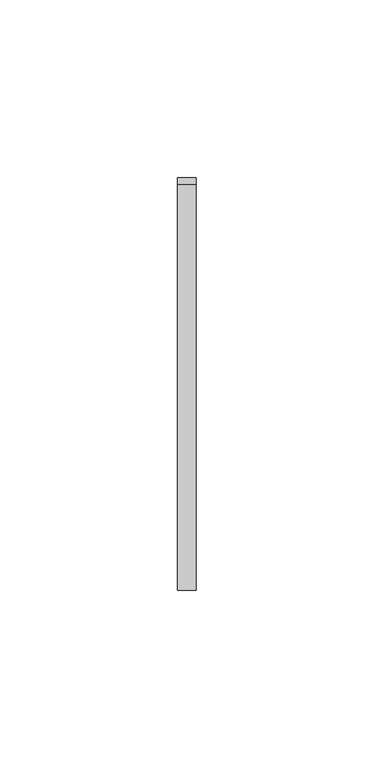
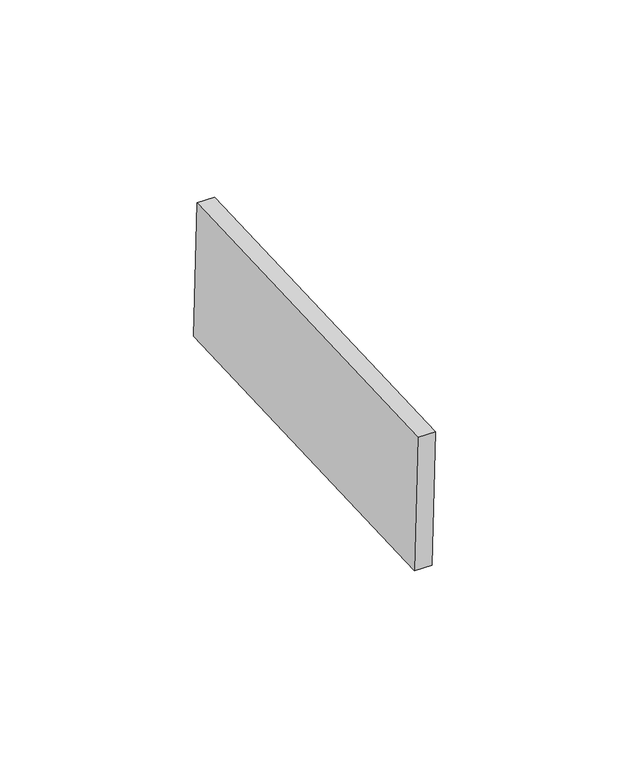
"""IFC4 building model written with IfcOpenShell, lengths in millimetres: proxy geometry, Inner panel:Inner panel:1:Inner panel:1 : Inner panel:Inner panel:300324:2:Inner panel:1:Inner panel:1 : Inner panel:Inner panel:300324:2 : Inner panel:Inner panel:1:Inner panel:1 : Inner panel:Inner panel:300324:300043:77 : Inner panel:Inner panel:1:Inner panel:1 : Inner panel:Inner panel:300324:2:Inner panel:1:Inner panel:1 : Inner panel:Inner panel:300324:2 : Inner panel:Inner panel:1:Inner panel:1 : Inner panel:Inner panel:300324:300043:308120."""

from ifc_helpers import new_model, si_unit, frame, origin, place, context, project, spatial, polyline, outline, extrude, source, transform, mapped, element, save


def generic_models_f36a7794(model_context):
    return source(origin(), model_context, "Body", "SweptSolid", [
        extrude(outline(polyline([(0.0, -114.3), (0.0, 0.0), (5.2138089, 0.0), (5.2138089, -114.3), (0.0, -114.3)])), frame((592717.395117, -578297.797364, 3981.6641254), z_axis=(0.0, -0.04163054471216399, 0.9991330730923527), x_axis=(-1.0, 0.0, 0.0)), (0.0, 0.0, 1.0), 43.2233908),
    ])


if __name__ == "__main__":
    model = new_model("IFC4")
    model_context = context("Model", 3, world=origin())
    ifc_project = project(units=[si_unit("LENGTHUNIT", "METRE", prefix="MILLI")], contexts=[model_context])
    site = spatial("IfcSite", under=ifc_project)
    building = spatial("IfcBuilding", under=site)
    placement = place(None, origin())
    generic_models_shape = generic_models_f36a7794(model_context)
    element("IfcBuildingElementProxy", 1, Name="Inner panel:Inner panel:1:Inner panel:1 : Inner panel:Inner panel:300324:2:Inner panel:1:Inner panel:1 : Inner panel:Inner panel:300324:2 : Inner panel:Inner panel:1:Inner panel:1 : Inner panel:Inner panel:300324:300043:77 : Inner panel:Inner panel:1:Inner panel:1 : Inner panel:Inner panel:300324:2:Inner panel:1:Inner panel:1 : Inner panel:Inner panel:300324:2 : Inner panel:Inner panel:1:Inner panel:1 : Inner panel:Inner panel:300324:300043:308120", ObjectType="Inner panel:Inner panel:1:Inner panel:1 : Inner panel:Inner panel:300324:2:Inner panel:1:Inner panel:1 : Inner panel:Inner panel:300324:2 : Inner panel:Inner panel:1:Inner panel:1 : Inner panel:Inner panel:300324:300043:77 : Inner panel:Inner panel:1:Inner panel:1 : Inner panel:Inner panel:300324:2:Inner panel:1:Inner panel:1 : Inner panel:Inner panel:300324:2 : Inner panel:Inner panel:1:Inner panel:1 : Inner panel:Inner panel:300324:300043:308120", at=placement, inside=building, context=model_context, shape_type="MappedRepresentation", body=[
        mapped(generic_models_shape, transform((0.0, 0.0, 0.0), x_axis=(1.0, 0.0, 0.0), y_axis=(0.0, 1.0, 0.0), z_axis=(0.0, 0.0, 1.0))),
    ])
    save(model, "model.ifc")

# Revit data of these elements
# Type "Inner panel:Inner panel:1:Inner panel:1 : Inner panel:Inner panel:300324:2:Inner panel:1:Inner panel:1 : Inner panel:Inner panel:300324:2 : Inner panel:Inner panel:1:Inner panel:1 : Inner panel:Inner panel:300324:300043:77 : Inner panel:Inner panel:1:Inner panel:1 : Inner panel:Inner panel:300324:2:Inner panel:1:Inner panel:1 : Inner panel:Inner panel:300324:2 : Inner panel:Inner panel:1:Inner panel:1 : Inner panel:Inner panel:300324:300043:308120"
#   NameOverride = "Inner panel:Inner panel:1:Inner panel:1 : Inner panel:Inner panel:300324:2:Inner panel:1:Inner panel:1 : Inner panel:Inner panel:300324:2 : Inner panel:Inner panel:1:Inner panel:1 : Inner panel:Inner panel:300324:300043:308120"
#   ObjectTypeOverride = "Inner panel:1:Inner panel:1 : Inner panel:Inner panel:300324:2 : Inner panel:Inner panel:1:Inner panel:1 : Inner panel:Inner panel:300324:300043"
#   Reference = "Inner panel"
#   Tag = "308120"
# Element 1 (IfcBuildingElementProxy, "Inner panel:Inner panel:1:Inner panel:1 : Inner panel:Inner panel:300324:2:Inner panel:1:Inner panel:1 : Inner panel:Inner panel:300324:2 : Inner panel:Inner panel:1:Inner panel:1 : Inner panel:Inner panel:300324:300043:77 : Inner panel:Inner panel:1:Inner panel:1 : Inner panel:Inner panel:300324:2:Inner panel:1:Inner panel:1 : Inner panel:Inner panel:300324:2 : Inner panel:Inner panel:1:Inner panel:1 : Inner panel:Inner panel:300324:300043:308120")
#   Materials on its faces: "SLIDING CLIP"
# Materials
#   "SLIDING CLIP": class "Generic", colour RGB 120 120 120, transparency 0, Cost = 0
